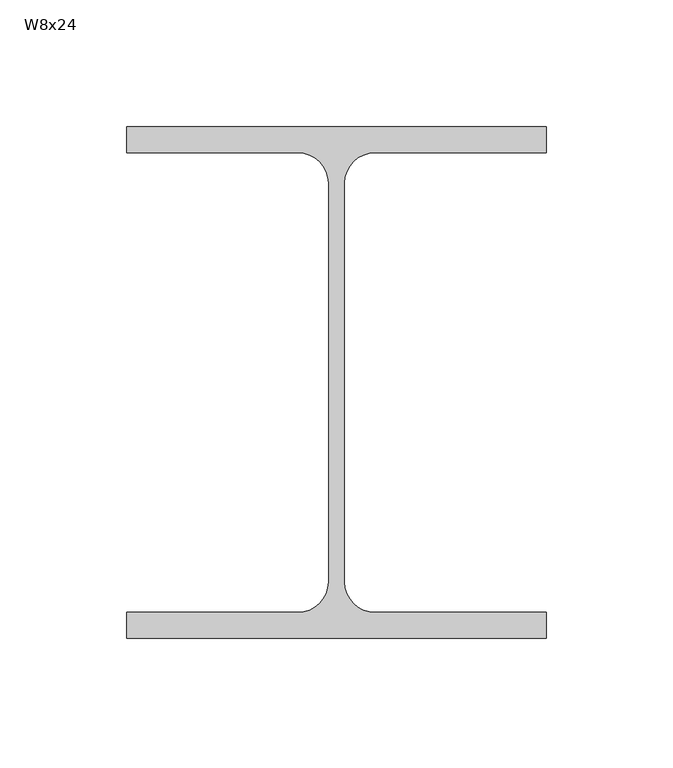
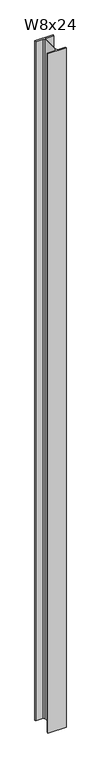
"""IFC4 building model written with IfcOpenShell, lengths in millimetres: column geometry, RME WF - Column : W8x24."""

from ifc_helpers import new_model, si_unit, point, frame, frame_2d, origin, place, context, project, spatial, polyline, circle_curve, trimmed, segment, composite_curve, outline, extrude, source, transform, mapped, element, save


def w8x24_47579d82(model_context):
    return source(origin(), model_context, "Body", "SweptSolid", [
        extrude(outline(composite_curve([segment(polyline([(82.55, 100.711), (82.55, 90.551), (15.1765, 90.551)]), True, "CONTINUOUS"), segment(trimmed(circle_curve(frame_2d((15.1765, 78.486)), 12.065), [point((15.1765, 90.551))], [point((3.1115, 78.486))], True, "CARTESIAN"), True, "CONTINUOUS"), segment(polyline([(3.1115, 78.486), (3.1115, -78.486)]), True, "CONTINUOUS"), segment(trimmed(circle_curve(frame_2d((15.1765, -78.486)), 12.065), [point((3.1115, -78.486))], [point((15.1765, -90.551))], True, "CARTESIAN"), True, "CONTINUOUS"), segment(polyline([(15.1765, -90.551), (82.55, -90.551), (82.55, -100.711), (-82.55, -100.711), (-82.55, -90.551), (-15.1765, -90.551)]), True, "CONTINUOUS"), segment(trimmed(circle_curve(frame_2d((-15.1765, -78.486)), 12.065), [point((-15.1765, -90.551))], [point((-3.1115, -78.486))], True, "CARTESIAN"), True, "CONTINUOUS"), segment(polyline([(-3.1115, -78.486), (-3.1115, 78.486)]), True, "CONTINUOUS"), segment(trimmed(circle_curve(frame_2d((-15.1765, 78.486)), 12.065), [point((-3.1115, 78.486))], [point((-15.1765, 90.551))], True, "CARTESIAN"), True, "CONTINUOUS"), segment(polyline([(-15.1765, 90.551), (-82.55, 90.551), (-82.55, 100.711), (82.55, 100.711)]), True, "CONTINUOUS")], self_intersect=False)), frame((0.0, 0.0, -304.8), z_axis=(0.0, 0.0, 1.0), x_axis=(1.0, 0.0, 0.0)), (0.0, 0.0, 1.0), 6489.7),
    ])


if __name__ == "__main__":
    model = new_model("IFC4")
    model_context = context("Model", 3, world=origin())
    ifc_project = project(units=[si_unit("LENGTHUNIT", "METRE", prefix="MILLI")], contexts=[model_context])
    site = spatial("IfcSite", under=ifc_project)
    building = spatial("IfcBuilding", under=site)
    placement = place(None, origin())
    w8x24_shape = w8x24_47579d82(model_context)
    element("IfcColumn", 1, ObjectType="RME WF - Column : W8x24", at=placement, inside=building, context=model_context, shape_type="MappedRepresentation", body=[
        mapped(w8x24_shape, transform((0.0, 0.0, 0.0), x_axis=(1.0, 0.0, 0.0), y_axis=(0.0, 1.0, 0.0), z_axis=(0.0, 0.0, 1.0))),
    ])
    save(model, "model.ifc")

# Revit data of these elements
# Type "RME WF - Column : W8x24"
#   Type Mark = "C1"
#   REINF TYPE [instance default] = ""
#   Nominal Size = "W16"
#   COL REMARKS [instance default] = ""
#   BP [instance default] = ""
#   Assembly Code = "B10"
#   W = 24
#   bf = 0' - 6 1/2"
#   d = 0' - 7.93"
#   k = 0' - 0 7/8"
#   kr = 0' - 0.475"
#   tf = 0' - 0.4"
#   tw = 0' - 0.245"
#   A = 0.0491667 SF
#   Structural Material [instance default] = Metal - Steel - ASTM A992
# Element 1 (IfcColumn, "RME WF - Column : W8x24")
#   Materials on its faces: "Metal - Steel - ASTM A992"
# Materials
#   "Metal - Steel - ASTM A992": class "Metal", colour RGB 255 128 0, transparency 0
